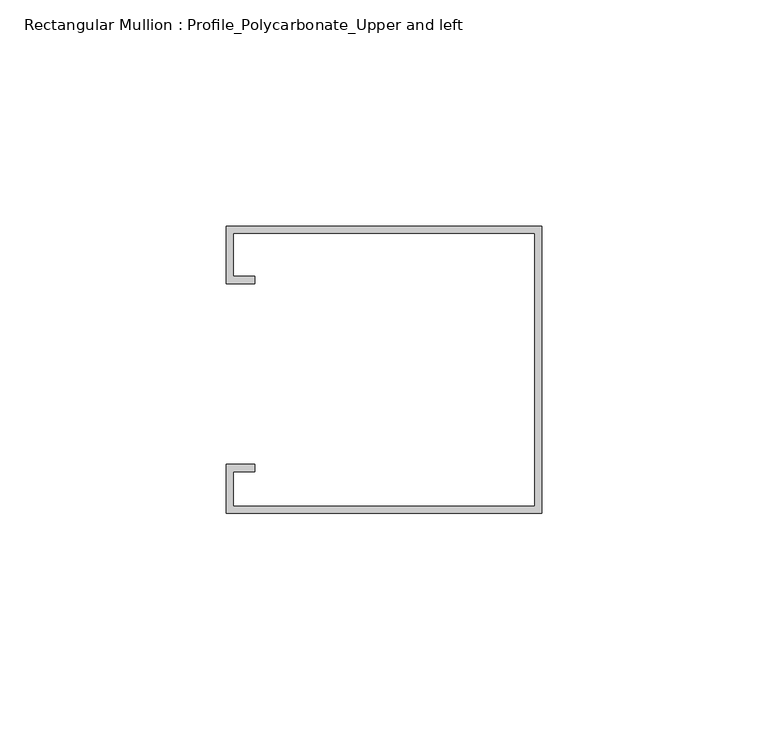
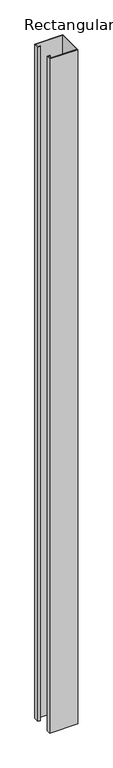
"""IFC4 building model written with IfcOpenShell, lengths in millimetres: member geometry, Rectangular Mullion : Profile_Polycarbonate_Upper and left."""

from ifc_helpers import new_model, si_unit, frame, origin, place, context, project, spatial, polyline, outline, extrude, source, transform, mapped, element, save


def rectangular_mullion_profile_polycarbonate_upper_and_left_a098d58f(model_context):
    return source(origin(), model_context, "Body", "SweptSolid", [
        extrude(outline(polyline([(0.0, 32.7), (0.0, -30.8), (-69.85, -30.8), (-69.85, -20.0), (-63.5, -20.0), (-63.5, -21.5875), (-68.2625, -21.5875), (-68.2625, -29.2125), (-1.5875, -29.2125), (-1.5875, 31.1125), (-68.2625, 31.1125), (-68.2625, 21.5875), (-63.5, 21.5875), (-63.5, 20.0), (-69.85, 20.0), (-69.85, 32.7), (0.0, 32.7)])), frame((0.0, 0.0, -1778.0), z_axis=(0.0, 0.0, 1.0), x_axis=(1.0, 0.0, 0.0)), (0.0, 0.0, 1.0), 1778.0),
    ])


if __name__ == "__main__":
    model = new_model("IFC4")
    model_context = context("Model", 3, world=origin())
    ifc_project = project(units=[si_unit("LENGTHUNIT", "METRE", prefix="MILLI")], contexts=[model_context])
    site = spatial("IfcSite", under=ifc_project)
    building = spatial("IfcBuilding", under=site)
    placement = place(None, origin())
    rectangular_mullion_profile_polycarbonate_upper_and_left_shape = rectangular_mullion_profile_polycarbonate_upper_and_left_a098d58f(model_context)
    element("IfcMember", 1, ObjectType="Rectangular Mullion : Profile_Polycarbonate_Upper and left", at=placement, inside=building, context=model_context, shape_type="MappedRepresentation", body=[
        mapped(rectangular_mullion_profile_polycarbonate_upper_and_left_shape, transform((0.0, 0.0, 0.0), x_axis=(1.0, 0.0, 0.0), y_axis=(0.0, 1.0, 0.0), z_axis=(0.0, 0.0, 1.0))),
    ])
    save(model, "model.ifc")

# Revit data of these elements
# Type "Rectangular Mullion : Profile_Polycarbonate_Upper and left"
#   built-in parameter 1007322 = 0.208333 (stored number, unit not read)
#   built-in parameter 1007321 = 0.00520833 (stored number, unit not read)
#   built-in parameter 1007320 = 0 (stored number, unit not read)
# Element 1 (IfcMember, "Rectangular Mullion : Profile_Polycarbonate_Upper and left")
#   Materials on its faces: "ALUMINUM PROFILE AT POLYCARBONATE PANEL"
# Materials
#   "ALUMINUM PROFILE AT POLYCARBONATE PANEL": class "Metal", colour RGB 244 244 244, transparency 0, Description = "Aluminum 6061", Cost = 0
